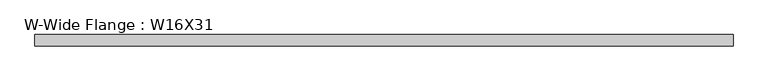
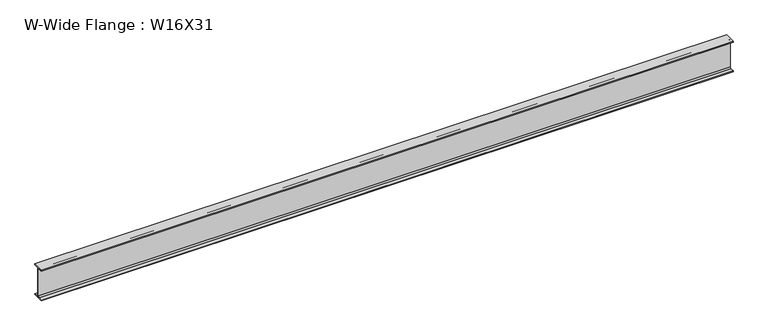
"""IFC4 building model written with IfcOpenShell, lengths in millimetres: beam geometry, W-Wide Flange : W16X31."""

from ifc_helpers import new_model, si_unit, point, frame, frame_2d, origin, place, context, project, spatial, polyline, circle_curve, trimmed, segment, composite_curve, outline, extrude, source, transform, mapped, element, save


def w_wide_flange_w16x31_d553f2e7(model_context):
    return source(origin(), model_context, "Body", "SweptSolid", [
        extrude(outline(composite_curve([segment(polyline([(70.231, -190.754), (70.231, -201.93), (-70.231, -201.93), (-70.231, -190.754), (-20.8915, -190.754)]), True, "CONTINUOUS"), segment(trimmed(circle_curve(frame_2d((-20.8915, -173.355)), 17.399), [point((-20.8915, -190.754))], [point((-3.4925, -173.355))], True, "CARTESIAN"), True, "CONTINUOUS"), segment(polyline([(-3.4925, -173.355), (-3.4925, 173.355)]), True, "CONTINUOUS"), segment(trimmed(circle_curve(frame_2d((-20.8915, 173.355)), 17.399), [point((-3.4925, 173.355))], [point((-20.8915, 190.754))], True, "CARTESIAN"), True, "CONTINUOUS"), segment(polyline([(-20.8915, 190.754), (-70.231, 190.754), (-70.231, 201.93), (70.231, 201.93), (70.231, 190.754), (20.8915, 190.754)]), True, "CONTINUOUS"), segment(trimmed(circle_curve(frame_2d((20.8915, 173.355)), 17.399), [point((20.8915, 190.754))], [point((3.4925, 173.355))], True, "CARTESIAN"), True, "CONTINUOUS"), segment(polyline([(3.4925, 173.355), (3.4925, -173.355)]), True, "CONTINUOUS"), segment(trimmed(circle_curve(frame_2d((20.8915, -173.355)), 17.399), [point((3.4925, -173.355))], [point((20.8915, -190.754))], True, "CARTESIAN"), True, "CONTINUOUS"), segment(polyline([(20.8915, -190.754), (70.231, -190.754)]), True, "CONTINUOUS")], self_intersect=False)), frame((-4336.669, 0.0, 0.0), z_axis=(1.0, 0.0, 0.0), x_axis=(0.0, 1.0, 0.0)), (0.0, 0.0, 1.0), 8673.338),
    ])


if __name__ == "__main__":
    model = new_model("IFC4")
    model_context = context("Model", 3, world=origin())
    ifc_project = project(units=[si_unit("LENGTHUNIT", "METRE", prefix="MILLI")], contexts=[model_context])
    site = spatial("IfcSite", under=ifc_project)
    building = spatial("IfcBuilding", under=site)
    placement = place(None, origin())
    w_wide_flange_w16x31_shape = w_wide_flange_w16x31_d553f2e7(model_context)
    element("IfcBeam", 1, ObjectType="W-Wide Flange : W16X31", at=placement, inside=building, context=model_context, shape_type="MappedRepresentation", body=[
        mapped(w_wide_flange_w16x31_shape, transform((0.0, 0.0, 0.0), x_axis=(1.0, 0.0, 0.0), y_axis=(0.0, 1.0, 0.0), z_axis=(0.0, 0.0, 1.0))),
    ])
    save(model, "model.ifc")

# Revit data of these elements
# Type "W-Wide Flange : W16X31"
#   Assembly Code = "B10"
#   W = 31
#   Start Extension Calculation [instance default] = 10' - 0"
#   Start Extension [instance default] = -0' - 0 1/2"
#   End Extension Calculation [instance default] = 10' - 0"
#   End Extension [instance default] = -0' - 0 1/2"
#   Length [instance default] = 5' - 0"
#   bf = 0' - 5.53"
#   d = 1' - 3.9"
#   k = 0' - 1 1/8"
#   k2 = 0' - 0.685"
#   tf = 0' - 0.44"
#   tw = 0' - 0.275"
#   A = 0.0634028 SF
#   Beam Material [instance default] = Metal - Steel - ASTM A992
# Element 1 (IfcBeam, "W-Wide Flange : W16X31")
#   Materials on its faces: "Metal - Steel - ASTM A992"
# Materials
#   "Metal - Steel - ASTM A992": class "Metal", colour RGB 128 0 0, transparency 0
